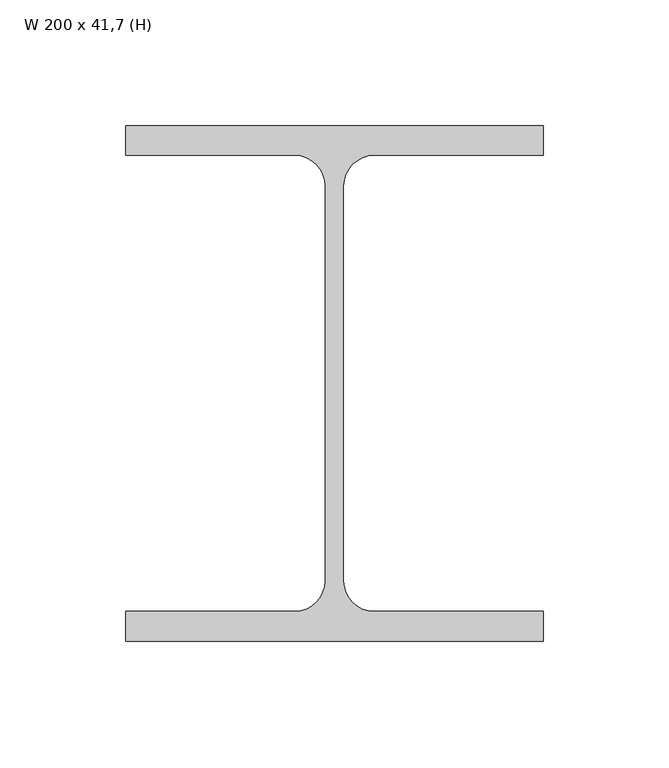
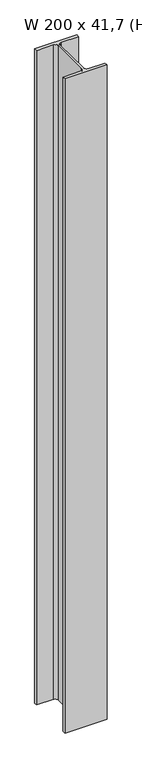
"""IFC4 building model written with IfcOpenShell, lengths in millimetres: column geometry, Pilar de Aço - H : W 200 x 41,7 (H)."""

from ifc_helpers import new_model, si_unit, point, frame_2d, origin, origin_with_axes, place, context, project, spatial, polyline, circle_curve, trimmed, segment, composite_curve, outline, extrude, source, transform, mapped, element, save


def w_200_x_41_7_h_22606ee6(model_context):
    return source(origin(), model_context, "Body", "SweptSolid", [
        extrude(outline(composite_curve([segment(polyline([(83.0, 102.5), (83.0, 90.7), (15.8, 90.7)]), True, "CONTINUOUS"), segment(trimmed(circle_curve(frame_2d((15.8, 78.5)), 12.2), [point((15.8, 90.7))], [point((3.6, 78.5))], True, "CARTESIAN"), True, "CONTINUOUS"), segment(polyline([(3.6, 78.5), (3.6, -78.5)]), True, "CONTINUOUS"), segment(trimmed(circle_curve(frame_2d((15.8, -78.5)), 12.2), [point((3.6, -78.5))], [point((15.8, -90.7))], True, "CARTESIAN"), True, "CONTINUOUS"), segment(polyline([(15.8, -90.7), (83.0, -90.7), (83.0, -102.5), (-83.0, -102.5), (-83.0, -90.7), (-15.8, -90.7)]), True, "CONTINUOUS"), segment(trimmed(circle_curve(frame_2d((-15.8, -78.5)), 12.2), [point((-15.8, -90.7))], [point((-3.6, -78.5))], True, "CARTESIAN"), True, "CONTINUOUS"), segment(polyline([(-3.6, -78.5), (-3.6, 78.5)]), True, "CONTINUOUS"), segment(trimmed(circle_curve(frame_2d((-15.8, 78.5)), 12.2), [point((-3.6, 78.5))], [point((-15.8, 90.7))], True, "CARTESIAN"), True, "CONTINUOUS"), segment(polyline([(-15.8, 90.7), (-83.0, 90.7), (-83.0, 102.5), (83.0, 102.5)]), True, "CONTINUOUS")], self_intersect=False)), origin_with_axes(), (0.0, 0.0, 1.0), 2720.0),
    ])


if __name__ == "__main__":
    model = new_model("IFC4")
    model_context = context("Model", 3, world=origin())
    ifc_project = project(units=[si_unit("LENGTHUNIT", "METRE", prefix="MILLI")], contexts=[model_context])
    site = spatial("IfcSite", under=ifc_project)
    building = spatial("IfcBuilding", under=site)
    placement = place(None, origin())
    w_200_x_41_7_h_shape = w_200_x_41_7_h_22606ee6(model_context)
    element("IfcColumn", 1, ObjectType="Pilar de Aço - H : W 200 x 41,7 (H)", at=placement, inside=building, context=model_context, shape_type="MappedRepresentation", body=[
        mapped(w_200_x_41_7_h_shape, transform((0.0, 0.0, 0.0), x_axis=(1.0, 0.0, 0.0), y_axis=(0.0, 1.0, 0.0), z_axis=(0.0, 0.0, 1.0))),
    ])
    save(model, "model.ifc")

# Revit data of these elements
# Type "Pilar de Aço - H : W 200 x 41,7 (H)"
#   SINAPI = ""
#   Área da seção = 53.5 m²
#   tw = 0.72 cm
#   tf = 1.18 cm
#   h = 18.14 cm
#   d' = 15.70 cm
#   d = 20.50 cm
#   bf = 16.60 cm
#   R = 1.22 cm
#   Massa Linear kg/m = 41.7
#   Aço = Metal - Aço 345MPa
#   Assembly Code = ""
# Materials
#   "Metal - Aço 345MPa": class "Metal", colour RGB 189 187 185, transparency 0, Cost = 0
